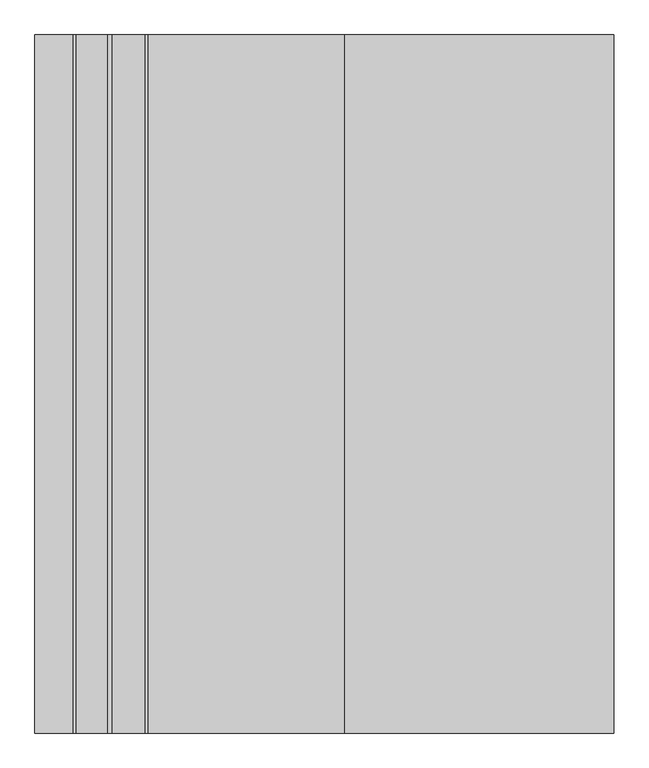
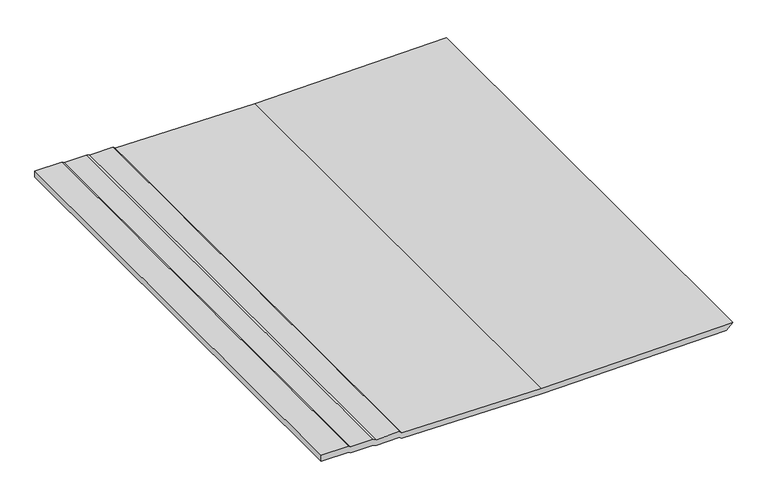
"""IFC4 building model written with IfcOpenShell, lengths in millimetres: proxy geometry, GRAVEL BALLAST002 15468 : GRAVEL BALLAST002 15468."""

import ifcopenshell
import ifcopenshell.guid

model = None  # the IFC model being written
_history = None  # IfcOwnerHistory: only IFC2X3 demands one
_inside = {}  # id of a spatial element -> (the spatial element, [elements in it])
_under = {}  # id of a project, library or spatial element -> (it, [spatial elements below it])
_declared = {}  # id of a project -> (the project, [libraries it declares])
_typed = {}  # id of a type object -> (the type object, [elements of that type])
_made_of = {}  # id of a material, layer set ... -> (it, [elements and type objects made of it])


def new_model(schema):
    """Start an empty IFC model of exactly this schema.

    Asked for "IFC4X3", IfcOpenShell would pick the latest addendum, in which some entities
    have other attributes; the version numbers below select the first issue.
    IFC2X3 requires an IfcOwnerHistory on every rooted entity: one is made here for all.
    """
    global model, _history
    if schema == "IFC4X3":
        model = ifcopenshell.file(schema_version=(4, 3, 0, 0))
    else:
        model = ifcopenshell.file(schema=schema)
    _inside.clear()
    _under.clear()
    _declared.clear()
    _typed.clear()
    _made_of.clear()
    _history = None
    if model.schema == "IFC2X3":
        org = make("IfcOrganization", Name="unknown")
        user = make(
            "IfcPersonAndOrganization",
            ThePerson=make("IfcPerson", FamilyName="unknown"),
            TheOrganization=org,
        )
        app = make(
            "IfcApplication",
            ApplicationDeveloper=org,
            Version="unknown",
            ApplicationFullName="unknown",
            ApplicationIdentifier="unknown",
        )
        _history = make(
            "IfcOwnerHistory",
            OwningUser=user,
            OwningApplication=app,
            ChangeAction="ADDED",
            CreationDate=0,
        )
    return model


def make(cls, **values):
    """One entity of the class cls with the attributes given. An attribute that is None is left unset."""
    return model.create_entity(
        cls, **{name: value for name, value in values.items() if value is not None}
    )


def rooted(cls, **values):
    """An entity with a GlobalId (a new one), such as an element, a storey or a relation."""
    return make(cls, GlobalId=ifcopenshell.guid.new(), OwnerHistory=_history, **values)


def si_unit(unit_type, name, prefix=None):
    """IfcSIUnit, for example si_unit("LENGTHUNIT", "METRE", prefix="MILLI")."""
    return make("IfcSIUnit", UnitType=unit_type, Prefix=prefix, Name=name)


def assignment(units):
    """IfcUnitAssignment: the units of a project."""
    return None if units is None else make("IfcUnitAssignment", Units=units)


def point(xyz):
    """IfcCartesianPoint."""
    return None if xyz is None else make("IfcCartesianPoint", Coordinates=xyz)


def direction(xyz):
    """IfcDirection."""
    return None if xyz is None else make("IfcDirection", DirectionRatios=xyz)


def frame(location, z_axis=None, x_axis=None):
    """IfcAxis2Placement3D, a coordinate frame: its origin and axes. An axis left out is left unset."""
    return make(
        "IfcAxis2Placement3D",
        Location=point(location),
        Axis=direction(z_axis),
        RefDirection=direction(x_axis),
    )


def origin():
    """The frame at (0, 0, 0) with its axes left unset."""
    return frame((0.0, 0.0, 0.0))


def place(relative_to, where):
    """IfcLocalPlacement: puts the frame where relative to a parent placement (None: the world)."""
    return make(
        "IfcLocalPlacement", PlacementRelTo=relative_to, RelativePlacement=where
    )


def context(
    kind, dimensions, precision=None, world=None, true_north=None, identifier=None
):
    """IfcGeometricRepresentationContext, for example the 3D "Model" context."""
    return make(
        "IfcGeometricRepresentationContext",
        ContextIdentifier=identifier,
        ContextType=kind,
        CoordinateSpaceDimension=dimensions,
        Precision=precision,
        WorldCoordinateSystem=world,
        TrueNorth=true_north,
    )


def project(units=None, contexts=None):
    """IfcProject with its units and contexts."""
    return rooted(
        "IfcProject",
        Name="project",
        RepresentationContexts=contexts,
        UnitsInContext=assignment(units),
    )


def spatial(cls, under=None, at=None, **own):
    """A site, building, storey or space (cls), placed at a placement, below another one or the project."""
    s = rooted(cls, ObjectPlacement=at, **own)
    if under is not None:
        _under.setdefault(under.id(), (under, []))[1].append(s)
    return s


def polyline(points):
    """IfcPolyline through the points."""
    return make("IfcPolyline", Points=[point(p) for p in points])


def outline(outer, holes=None, kind="AREA"):
    """IfcArbitraryClosedProfileDef: a profile drawn as a closed curve; with holes, ...WithVoids."""
    if holes is None:
        return make("IfcArbitraryClosedProfileDef", ProfileType=kind, OuterCurve=outer)
    return make(
        "IfcArbitraryProfileDefWithVoids",
        ProfileType=kind,
        OuterCurve=outer,
        InnerCurves=holes,
    )


def extrude(swept, where, along, depth):
    """IfcExtrudedAreaSolid: the profile swept, set in the frame where, extruded along a direction by depth."""
    return make(
        "IfcExtrudedAreaSolid",
        SweptArea=swept,
        Position=where,
        ExtrudedDirection=direction(along),
        Depth=depth,
    )


def shape(context_of_items, identifier, shape_type, items):
    """IfcShapeRepresentation: the items that make up one representation, for example the "Body"."""
    return make(
        "IfcShapeRepresentation",
        ContextOfItems=context_of_items,
        RepresentationIdentifier=identifier,
        RepresentationType=shape_type,
        Items=items,
    )


def source(mapping_origin, context_of_items, identifier, shape_type, items):
    """IfcRepresentationMap: a shape defined once, which mapped items show again and again."""
    return make(
        "IfcRepresentationMap",
        MappingOrigin=mapping_origin,
        MappedRepresentation=shape(context_of_items, identifier, shape_type, items),
    )


def transform(
    local_origin,
    x_axis=None,
    y_axis=None,
    z_axis=None,
    scale=None,
    scale2=None,
    scale3=None,
    uniform=True,
):
    """IfcCartesianTransformationOperator3D, or its non-uniform kind. x_axis, y_axis, z_axis: its Axis1, 2, 3."""
    if uniform:
        return make(
            "IfcCartesianTransformationOperator3D",
            Axis1=direction(x_axis),
            Axis2=direction(y_axis),
            LocalOrigin=point(local_origin),
            Scale=scale,
            Axis3=direction(z_axis),
        )
    return make(
        "IfcCartesianTransformationOperator3DnonUniform",
        Axis1=direction(x_axis),
        Axis2=direction(y_axis),
        LocalOrigin=point(local_origin),
        Scale=scale,
        Axis3=direction(z_axis),
        Scale2=scale2,
        Scale3=scale3,
    )


def mapped(mapping_source, mapping_target):
    """IfcMappedItem: shows the shape of a source again, moved by a transform."""
    return make(
        "IfcMappedItem", MappingSource=mapping_source, MappingTarget=mapping_target
    )


def made_of(thing, what):
    """Note that an element or type object is made of a material, layer set ...; save() writes the relation."""
    if what is not None:
        _made_of.setdefault(what.id(), (what, []))[1].append(thing)
    return thing


def element(
    cls,
    number,
    at=None,
    inside=None,
    cuts=None,
    type_object=None,
    material=None,
    context=None,
    identifier="Body",
    shape_type=None,
    held_by="IfcProductDefinitionShape",
    body=None,
    shapes=None,
    **own,
):
    """One element of the class cls, such as IfcWall. Its Tag is "e" and its number.

    at: its placement. inside: the storey or other place that contains it. cuts: it is an
    opening in that element (IfcRelVoidsElement). A single representation is given by context,
    identifier, shape_type and body (its items); several are given by shapes. held_by: the class
    of the entity that holds the representations. save() writes the other relations.
    """
    e = rooted(cls, Tag="e%d" % number, ObjectPlacement=at, **own)
    if body is not None:
        shapes = [shape(context, identifier, shape_type, body)]
    if shapes is not None:
        e.Representation = make(held_by, Representations=shapes)
    if inside is not None:
        _inside.setdefault(inside.id(), (inside, []))[1].append(e)
    if cuts is not None:
        rooted(
            "IfcRelVoidsElement", RelatingBuildingElement=cuts, RelatedOpeningElement=e
        )
    if type_object is not None:
        _typed.setdefault(type_object.id(), (type_object, []))[1].append(e)
    return made_of(e, material)


def aggregate(whole, parts):
    """IfcRelAggregates: a whole, such as a stair, and the parts it consists of."""
    return rooted("IfcRelAggregates", RelatingObject=whole, RelatedObjects=parts)


def save(model, path):
    """Write the relations noted so far, then the file.

    IfcRelAggregates (storeys below a building ...), IfcRelContainedInSpatialStructure (elements
    in a storey), IfcRelDefinesByType, IfcRelAssociatesMaterial and IfcRelDeclares: one each for
    every whole, place, type object, material and project.
    """
    for whole, parts in _under.values():
        aggregate(whole, parts)
    for where, things in _inside.values():
        rooted(
            "IfcRelContainedInSpatialStructure",
            RelatedElements=things,
            RelatingStructure=where,
        )
    for kind, things in _typed.values():
        rooted("IfcRelDefinesByType", RelatedObjects=things, RelatingType=kind)
    for what, things in _made_of.values():
        rooted("IfcRelAssociatesMaterial", RelatedObjects=things, RelatingMaterial=what)
    for by, libraries in _declared.values():
        rooted("IfcRelDeclares", RelatingContext=by, RelatedDefinitions=libraries)
    model.write(path)


def generic_models_deb63274(model_context):
    return source(origin(), model_context, "Body", "SweptSolid", [
        extrude(outline(polyline([(40274.2359465, -2672.3662777), (40269.9546965, -2663.6558285), (40269.9546965, -2573.0689144), (40264.2272345, -2560.2242751), (40265.8726652, -2466.2725277), (40258.462509, -2457.9990902), (40250.243759, -1894.9286556), (40261.546875, -1149.4367676), (40286.2851563, -1123.4630127), (40274.9820403, -1894.9286556), (40283.2007903, -2457.9990902), (40290.6109465, -2466.2725277), (40288.9655158, -2560.2242751), (40294.6929778, -2573.0689144), (40294.6929778, -2663.6558285), (40298.9742278, -2672.3662777), (40298.9742278, -2781.8657894), (40274.2359465, -2781.8657894), (40274.2359465, -2672.3662777)])), frame((0.0, -1052.6406573, 0.0), z_axis=(0.0, 1.0, 0.0), x_axis=(0.0, 0.0, 1.0)), (0.0, 0.0, 1.0), 2000.0),
    ])


if __name__ == "__main__":
    model = new_model("IFC4")
    model_context = context("Model", 3, world=origin())
    ifc_project = project(units=[si_unit("LENGTHUNIT", "METRE", prefix="MILLI")], contexts=[model_context])
    site = spatial("IfcSite", under=ifc_project)
    building = spatial("IfcBuilding", under=site)
    placement = place(None, origin())
    generic_models_shape = generic_models_deb63274(model_context)
    element("IfcBuildingElementProxy", 1, Name="GRAVEL BALLAST002 15468 : GRAVEL BALLAST002 15468", ObjectType="GRAVEL BALLAST002 15468 : GRAVEL BALLAST002 15468", at=placement, inside=building, context=model_context, shape_type="MappedRepresentation", body=[
        mapped(generic_models_shape, transform((0.0, 0.0, 0.0), x_axis=(1.0, 0.0, 0.0), y_axis=(0.0, 1.0, 0.0), z_axis=(0.0, 0.0, 1.0))),
    ])
    save(model, "model.ifc")

# Revit data of these elements
# Type "GRAVEL BALLAST002 15468 : GRAVEL BALLAST002 15468"
#   NameOverride = "GRAVEL BALLAST002"
# Element 1 (IfcBuildingElementProxy, "GRAVEL BALLAST002 15468 : GRAVEL BALLAST002 15468")
#   Materials on its faces: "GRAVEL BALLAST"
# Materials
#   "GRAVEL BALLAST": class "Unassigned", colour RGB 128 128 128, transparency 0, Cost = 0
